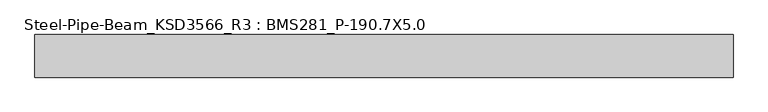
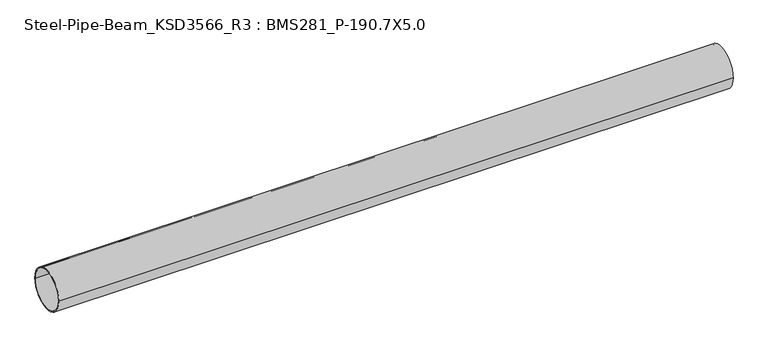
"""IFC4 building model written with IfcOpenShell, lengths in millimetres: member geometry, Steel-Pipe-Beam_KSD3566_R3 : BMS281_P-190.7X5.0."""

from ifc_helpers import new_model, si_unit, point, frame, origin, origin_2d, place, context, project, spatial, circle_curve, trimmed, segment, composite_curve, outline, extrude, source, transform, mapped, element, save


def steel_pipe_beam_ksd3566_r3_bms281_p_190_7x5_0_63a6a090(model_context):
    return source(origin(), model_context, "Body", "SweptSolid", [
        extrude(outline(composite_curve([segment(trimmed(circle_curve(origin_2d(), 95.35), [point((-95.35, 0.0))], [point((95.35, 0.0))], False, "CARTESIAN"), True, "CONTINUOUS"), segment(trimmed(circle_curve(origin_2d(), 95.35), [point((95.35, 0.0))], [point((-95.35, 0.0))], False, "CARTESIAN"), True, "CONTINUOUS")], self_intersect=False), holes=[composite_curve([segment(trimmed(circle_curve(origin_2d(), 90.35), [point((90.35, 0.0))], [point((-90.35, 0.0))], True, "CARTESIAN"), True, "CONTINUOUS"), segment(trimmed(circle_curve(origin_2d(), 90.35), [point((-90.35, 0.0))], [point((90.35, 0.0))], True, "CARTESIAN"), True, "CONTINUOUS")], self_intersect=False)]), frame((-1634.1462761, 0.0, 0.0), z_axis=(1.0, 0.0, 0.0), x_axis=(0.0, 1.0, 0.0)), (0.0, 0.0, 1.0), 3121.8221627),
    ])


if __name__ == "__main__":
    model = new_model("IFC4")
    model_context = context("Model", 3, world=origin())
    ifc_project = project(units=[si_unit("LENGTHUNIT", "METRE", prefix="MILLI")], contexts=[model_context])
    site = spatial("IfcSite", under=ifc_project)
    building = spatial("IfcBuilding", under=site)
    placement = place(None, origin())
    steel_pipe_beam_ksd3566_r3_bms281_p_190_7x5_0_shape = steel_pipe_beam_ksd3566_r3_bms281_p_190_7x5_0_63a6a090(model_context)
    element("IfcMember", 1, ObjectType="Steel-Pipe-Beam_KSD3566_R3 : BMS281_P-190.7X5.0", at=placement, inside=building, context=model_context, shape_type="MappedRepresentation", body=[
        mapped(steel_pipe_beam_ksd3566_r3_bms281_p_190_7x5_0_shape, transform((0.0, 0.0, 0.0), x_axis=(1.0, 0.0, 0.0), y_axis=(0.0, 1.0, 0.0), z_axis=(0.0, 0.0, 1.0))),
    ])
    save(model, "model.ifc")

# Revit data of these elements
# Type "Steel-Pipe-Beam_KSD3566_R3 : BMS281_P-190.7X5.0"
#   Keynote = "P-190.7X5.0"
#   SteelWeight = "Light"
#   t = 0.0050 m
#   Surface Area = 0.599102 m²/m
#   Section Area = 29.1697 cm²
#   Mass per Unit Length = 22.8982 kg/m
#   Length [instance default] = 1.5000 m
#   D = 0.1907 m
#   hec_material4 [instance default] = none
#   hec_material3 [instance default] = none
#   hec_material2 [instance default] = none
#   hec_material1 [instance default] = none
#   Structural Material [instance default] = Steel, 45-345
#   Assembly Code = ""
# Element 1 (IfcMember, "Steel-Pipe-Beam_KSD3566_R3 : BMS281_P-190.7X5.0")
#   Structural Material = none
# Materials
#   "Steel, 45-345": class "Metal", colour RGB 189 187 185, transparency 0, Description = "Steel 345 MPa", Cost = 0
